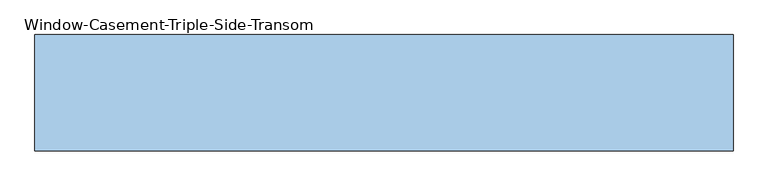
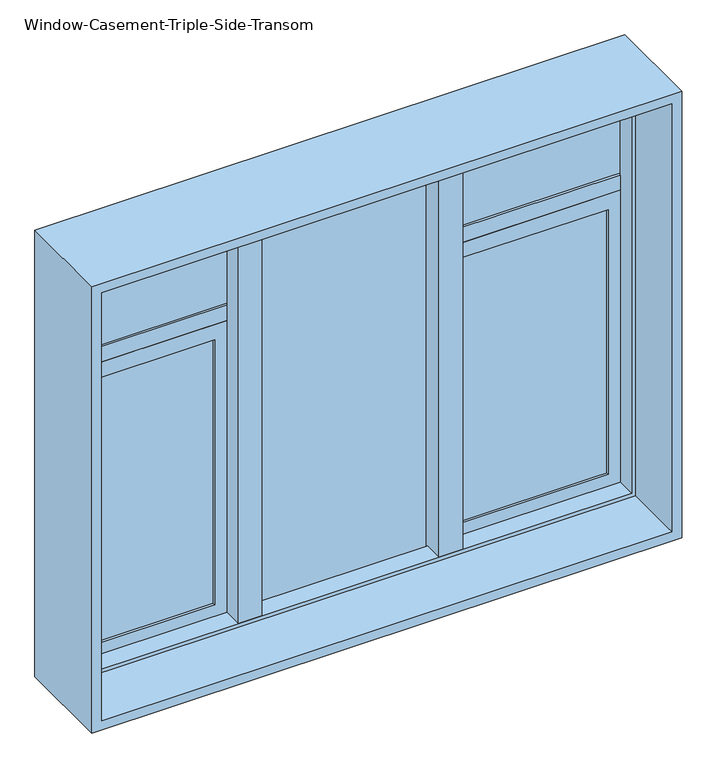
"""IFC4 building model written with IfcOpenShell, lengths in millimetres: window geometry, Window-Casement-Triple-Side-Transom : 5'*4' Window."""

import ifcopenshell
import ifcopenshell.guid

model = None  # the IFC model being written
_history = None  # IfcOwnerHistory: only IFC2X3 demands one
_inside = {}  # id of a spatial element -> (the spatial element, [elements in it])
_under = {}  # id of a project, library or spatial element -> (it, [spatial elements below it])
_declared = {}  # id of a project -> (the project, [libraries it declares])
_typed = {}  # id of a type object -> (the type object, [elements of that type])
_made_of = {}  # id of a material, layer set ... -> (it, [elements and type objects made of it])


def new_model(schema):
    """Start an empty IFC model of exactly this schema.

    Asked for "IFC4X3", IfcOpenShell would pick the latest addendum, in which some entities
    have other attributes; the version numbers below select the first issue.
    IFC2X3 requires an IfcOwnerHistory on every rooted entity: one is made here for all.
    """
    global model, _history
    if schema == "IFC4X3":
        model = ifcopenshell.file(schema_version=(4, 3, 0, 0))
    else:
        model = ifcopenshell.file(schema=schema)
    _inside.clear()
    _under.clear()
    _declared.clear()
    _typed.clear()
    _made_of.clear()
    _history = None
    if model.schema == "IFC2X3":
        org = make("IfcOrganization", Name="unknown")
        user = make(
            "IfcPersonAndOrganization",
            ThePerson=make("IfcPerson", FamilyName="unknown"),
            TheOrganization=org,
        )
        app = make(
            "IfcApplication",
            ApplicationDeveloper=org,
            Version="unknown",
            ApplicationFullName="unknown",
            ApplicationIdentifier="unknown",
        )
        _history = make(
            "IfcOwnerHistory",
            OwningUser=user,
            OwningApplication=app,
            ChangeAction="ADDED",
            CreationDate=0,
        )
    return model


def make(cls, **values):
    """One entity of the class cls with the attributes given. An attribute that is None is left unset."""
    return model.create_entity(
        cls, **{name: value for name, value in values.items() if value is not None}
    )


def rooted(cls, **values):
    """An entity with a GlobalId (a new one), such as an element, a storey or a relation."""
    return make(cls, GlobalId=ifcopenshell.guid.new(), OwnerHistory=_history, **values)


def si_unit(unit_type, name, prefix=None):
    """IfcSIUnit, for example si_unit("LENGTHUNIT", "METRE", prefix="MILLI")."""
    return make("IfcSIUnit", UnitType=unit_type, Prefix=prefix, Name=name)


def assignment(units):
    """IfcUnitAssignment: the units of a project."""
    return None if units is None else make("IfcUnitAssignment", Units=units)


def point(xyz):
    """IfcCartesianPoint."""
    return None if xyz is None else make("IfcCartesianPoint", Coordinates=xyz)


def direction(xyz):
    """IfcDirection."""
    return None if xyz is None else make("IfcDirection", DirectionRatios=xyz)


def frame(location, z_axis=None, x_axis=None):
    """IfcAxis2Placement3D, a coordinate frame: its origin and axes. An axis left out is left unset."""
    return make(
        "IfcAxis2Placement3D",
        Location=point(location),
        Axis=direction(z_axis),
        RefDirection=direction(x_axis),
    )


def origin():
    """The frame at (0, 0, 0) with its axes left unset."""
    return frame((0.0, 0.0, 0.0))


def place(relative_to, where):
    """IfcLocalPlacement: puts the frame where relative to a parent placement (None: the world)."""
    return make(
        "IfcLocalPlacement", PlacementRelTo=relative_to, RelativePlacement=where
    )


def context(
    kind, dimensions, precision=None, world=None, true_north=None, identifier=None
):
    """IfcGeometricRepresentationContext, for example the 3D "Model" context."""
    return make(
        "IfcGeometricRepresentationContext",
        ContextIdentifier=identifier,
        ContextType=kind,
        CoordinateSpaceDimension=dimensions,
        Precision=precision,
        WorldCoordinateSystem=world,
        TrueNorth=true_north,
    )


def project(units=None, contexts=None):
    """IfcProject with its units and contexts."""
    return rooted(
        "IfcProject",
        Name="project",
        RepresentationContexts=contexts,
        UnitsInContext=assignment(units),
    )


def spatial(cls, under=None, at=None, **own):
    """A site, building, storey or space (cls), placed at a placement, below another one or the project."""
    s = rooted(cls, ObjectPlacement=at, **own)
    if under is not None:
        _under.setdefault(under.id(), (under, []))[1].append(s)
    return s


def polyline(points):
    """IfcPolyline through the points."""
    return make("IfcPolyline", Points=[point(p) for p in points])


def outline(outer, holes=None, kind="AREA"):
    """IfcArbitraryClosedProfileDef: a profile drawn as a closed curve; with holes, ...WithVoids."""
    if holes is None:
        return make("IfcArbitraryClosedProfileDef", ProfileType=kind, OuterCurve=outer)
    return make(
        "IfcArbitraryProfileDefWithVoids",
        ProfileType=kind,
        OuterCurve=outer,
        InnerCurves=holes,
    )


def extrude(swept, where, along, depth):
    """IfcExtrudedAreaSolid: the profile swept, set in the frame where, extruded along a direction by depth."""
    return make(
        "IfcExtrudedAreaSolid",
        SweptArea=swept,
        Position=where,
        ExtrudedDirection=direction(along),
        Depth=depth,
    )


def faces_of(points, faces, orient=None, outer=None):
    """IfcFace entities. A face is a list of loops; a loop is a list of indices into points, from 0.

    orient and outer hold one flag for each loop. By default every Orientation is true, the
    first loop of a face is its IfcFaceOuterBound and the others are IfcFaceBound.
    """
    made = []
    for i, loops in enumerate(faces):
        bounds = []
        for j, loop in enumerate(loops):
            is_outer = j == 0 if outer is None else outer[i][j]
            bounds.append(
                make(
                    "IfcFaceOuterBound" if is_outer else "IfcFaceBound",
                    Bound=make("IfcPolyLoop", Polygon=[points[k] for k in loop]),
                    Orientation=True if orient is None else orient[i][j],
                )
            )
        made.append(make("IfcFace", Bounds=bounds))
    return made


def faceted_brep(points, faces, orient=None, outer=None, voids=None):
    """IfcFacetedBrep: a solid bounded by flat faces; with voids (closed shells), ...WithVoids."""
    shared = [point(p) for p in points]
    hull = make("IfcClosedShell", CfsFaces=faces_of(shared, faces, orient, outer))
    if voids is None:
        return make("IfcFacetedBrep", Outer=hull)
    return make(
        "IfcFacetedBrepWithVoids",
        Outer=hull,
        Voids=[
            make(cls, CfsFaces=faces_of(shared, fs, o, b)) for cls, fs, o, b in voids
        ],
    )


def shape(context_of_items, identifier, shape_type, items):
    """IfcShapeRepresentation: the items that make up one representation, for example the "Body"."""
    return make(
        "IfcShapeRepresentation",
        ContextOfItems=context_of_items,
        RepresentationIdentifier=identifier,
        RepresentationType=shape_type,
        Items=items,
    )


def source(mapping_origin, context_of_items, identifier, shape_type, items):
    """IfcRepresentationMap: a shape defined once, which mapped items show again and again."""
    return make(
        "IfcRepresentationMap",
        MappingOrigin=mapping_origin,
        MappedRepresentation=shape(context_of_items, identifier, shape_type, items),
    )


def transform(
    local_origin,
    x_axis=None,
    y_axis=None,
    z_axis=None,
    scale=None,
    scale2=None,
    scale3=None,
    uniform=True,
):
    """IfcCartesianTransformationOperator3D, or its non-uniform kind. x_axis, y_axis, z_axis: its Axis1, 2, 3."""
    if uniform:
        return make(
            "IfcCartesianTransformationOperator3D",
            Axis1=direction(x_axis),
            Axis2=direction(y_axis),
            LocalOrigin=point(local_origin),
            Scale=scale,
            Axis3=direction(z_axis),
        )
    return make(
        "IfcCartesianTransformationOperator3DnonUniform",
        Axis1=direction(x_axis),
        Axis2=direction(y_axis),
        LocalOrigin=point(local_origin),
        Scale=scale,
        Axis3=direction(z_axis),
        Scale2=scale2,
        Scale3=scale3,
    )


def mapped(mapping_source, mapping_target):
    """IfcMappedItem: shows the shape of a source again, moved by a transform."""
    return make(
        "IfcMappedItem", MappingSource=mapping_source, MappingTarget=mapping_target
    )


def made_of(thing, what):
    """Note that an element or type object is made of a material, layer set ...; save() writes the relation."""
    if what is not None:
        _made_of.setdefault(what.id(), (what, []))[1].append(thing)
    return thing


def element(
    cls,
    number,
    at=None,
    inside=None,
    cuts=None,
    type_object=None,
    material=None,
    context=None,
    identifier="Body",
    shape_type=None,
    held_by="IfcProductDefinitionShape",
    body=None,
    shapes=None,
    **own,
):
    """One element of the class cls, such as IfcWall. Its Tag is "e" and its number.

    at: its placement. inside: the storey or other place that contains it. cuts: it is an
    opening in that element (IfcRelVoidsElement). A single representation is given by context,
    identifier, shape_type and body (its items); several are given by shapes. held_by: the class
    of the entity that holds the representations. save() writes the other relations.
    """
    e = rooted(cls, Tag="e%d" % number, ObjectPlacement=at, **own)
    if body is not None:
        shapes = [shape(context, identifier, shape_type, body)]
    if shapes is not None:
        e.Representation = make(held_by, Representations=shapes)
    if inside is not None:
        _inside.setdefault(inside.id(), (inside, []))[1].append(e)
    if cuts is not None:
        rooted(
            "IfcRelVoidsElement", RelatingBuildingElement=cuts, RelatedOpeningElement=e
        )
    if type_object is not None:
        _typed.setdefault(type_object.id(), (type_object, []))[1].append(e)
    return made_of(e, material)


def aggregate(whole, parts):
    """IfcRelAggregates: a whole, such as a stair, and the parts it consists of."""
    return rooted("IfcRelAggregates", RelatingObject=whole, RelatedObjects=parts)


def save(model, path):
    """Write the relations noted so far, then the file.

    IfcRelAggregates (storeys below a building ...), IfcRelContainedInSpatialStructure (elements
    in a storey), IfcRelDefinesByType, IfcRelAssociatesMaterial and IfcRelDeclares: one each for
    every whole, place, type object, material and project.
    """
    for whole, parts in _under.values():
        aggregate(whole, parts)
    for where, things in _inside.values():
        rooted(
            "IfcRelContainedInSpatialStructure",
            RelatedElements=things,
            RelatingStructure=where,
        )
    for kind, things in _typed.values():
        rooted("IfcRelDefinesByType", RelatedObjects=things, RelatingType=kind)
    for what, things in _made_of.values():
        rooted("IfcRelAssociatesMaterial", RelatedObjects=things, RelatingMaterial=what)
    for by, libraries in _declared.values():
        rooted("IfcRelDeclares", RelatingContext=by, RelatedDefinitions=libraries)
    model.write(path)


def window_casement_triple_side_transom_94e0c3a0(model_context):
    return source(origin(), model_context, "Body", "SolidModel", [
        faceted_brep([(-736.6, 85.725, 1955.8), (-736.6, 127.0, 1955.8), (736.6, 127.0, 1955.8), (736.6, 85.725, 1955.8), (-726.4796875, 34.925, 1945.6796875), (-726.4796875, 85.725, 1945.6796875), (726.4796875, 85.725, 1945.6796875), (726.4796875, 34.925, 1945.6796875), (-736.6, -127.0, 1955.8), (-736.6, 34.925, 1955.8), (736.6, 34.925, 1955.8), (736.6, -127.0, 1955.8), (-762.0, 127.0, 1981.2), (-762.0, -127.0, 1981.2), (762.0, -127.0, 1981.2), (762.0, 127.0, 1981.2), (736.6, 127.0, 787.4), (736.6, 85.725, 787.4), (726.4796875, 85.725, 797.5203125), (726.4796875, 34.925, 797.5203125), (736.6, 34.925, 787.4), (736.6, -127.0, 787.4), (762.0, -127.0, 762.0), (762.0, 127.0, 762.0), (-736.6, 127.0, 787.4), (-736.6, 85.725, 787.4), (-726.4796875, 85.725, 797.5203125), (-726.4796875, 34.925, 797.5203125), (-736.6, 34.925, 787.4), (-736.6, -127.0, 787.4), (-762.0, -127.0, 762.0), (-762.0, 127.0, 762.0)], [[[0, 1, 2, 3]], [[4, 5, 6, 7]], [[8, 9, 10, 11]], [[12, 13, 14, 15]], [[3, 2, 16, 17]], [[7, 6, 18, 19]], [[11, 10, 20, 21]], [[15, 14, 22, 23]], [[17, 16, 24, 25]], [[19, 18, 26, 27]], [[21, 20, 28, 29]], [[23, 22, 30, 31]], [[25, 24, 1, 0]], [[3, 17, 25, 0], [5, 26, 18, 6]], [[27, 26, 5, 4]], [[9, 28, 20, 10], [7, 19, 27, 4]], [[29, 28, 9, 8]], [[13, 30, 22, 14], [11, 21, 29, 8]], [[31, 30, 13, 12]], [[15, 23, 31, 12], [1, 24, 16, 2]]]),
        extrude(outline(polyline([(-228.6, 123.825), (-228.6, 34.925), (-289.5203125, 34.925), (-289.5203125, 85.725), (-279.4, 85.725), (-279.4, 123.825), (-228.6, 123.825)])), frame((0.0, 0.0, 787.4), z_axis=(0.0, 0.0, 1.0), x_axis=(1.0, 0.0, 0.0)), (0.0, 0.0, 1.0), 1168.4),
        extrude(outline(polyline([(279.4, 123.825), (279.4, 85.725), (289.5203125, 85.725), (289.5203125, 34.925), (228.6, 34.925), (228.6, 123.825), (279.4, 123.825)])), frame((0.0, 0.0, 787.4), z_axis=(0.0, 0.0, 1.0), x_axis=(1.0, 0.0, 0.0)), (0.0, 0.0, 1.0), 1168.4),
        extrude(outline(polyline([(1594.5048438, 279.4), (787.4, 279.4), (787.4, 736.6), (1594.5048438, 736.6), (1594.5048438, 279.4)]), holes=[polyline([(1552.6345313, 694.7296875), (829.2703125, 694.7296875), (829.2703125, 321.2703125), (1552.6345313, 321.2703125), (1552.6345313, 694.7296875)])]), frame((0.0, 85.725, 0.0), z_axis=(0.0, 1.0, 0.0), x_axis=(0.0, 0.0, 1.0)), (0.0, 0.0, 1.0), 31.75),
        extrude(outline(polyline([(1594.5048438, -736.6), (787.4, -736.6), (787.4, -279.4), (1594.5048438, -279.4), (1594.5048438, -736.6)]), holes=[polyline([(1552.6345313, -321.2703125), (829.2703125, -321.2703125), (829.2703125, -694.7296875), (1552.6345313, -694.7296875), (1552.6345313, -321.2703125)])]), frame((0.0, 85.725, 0.0), z_axis=(0.0, 1.0, 0.0), x_axis=(0.0, 0.0, 1.0)), (0.0, 0.0, 1.0), 31.75),
        extrude(outline(polyline([(-321.2703125, 111.125), (-321.2703125, 104.775), (-694.7296875, 104.775), (-694.7296875, 111.125), (-321.2703125, 111.125)])), frame((0.0, 0.0, 829.2703125), z_axis=(0.0, 0.0, 1.0), x_axis=(1.0, 0.0, 0.0)), (0.0, 0.0, 1.0), 723.3642188),
        extrude(outline(polyline([(-321.2703125, 98.425), (-321.2703125, 92.075), (-694.7296875, 92.075), (-694.7296875, 98.425), (-321.2703125, 98.425)])), frame((0.0, 0.0, 829.2703125), z_axis=(0.0, 0.0, 1.0), x_axis=(1.0, 0.0, 0.0)), (0.0, 0.0, 1.0), 723.3642188),
        extrude(outline(polyline([(694.7296875, 111.125), (694.7296875, 104.775), (321.2703125, 104.775), (321.2703125, 111.125), (694.7296875, 111.125)])), frame((0.0, 0.0, 829.2703125), z_axis=(0.0, 0.0, 1.0), x_axis=(1.0, 0.0, 0.0)), (0.0, 0.0, 1.0), 723.3642188),
        extrude(outline(polyline([(694.7296875, 98.425), (694.7296875, 92.075), (321.2703125, 92.075), (321.2703125, 98.425), (694.7296875, 98.425)])), frame((0.0, 0.0, 829.2703125), z_axis=(0.0, 0.0, 1.0), x_axis=(1.0, 0.0, 0.0)), (0.0, 0.0, 1.0), 723.3642188),
        extrude(outline(polyline([(736.6, 117.475), (736.6, 85.725), (279.4, 85.725), (279.4, 117.475), (736.6, 117.475)])), frame((0.0, 0.0, 1594.5048438), z_axis=(0.0, 0.0, 1.0), x_axis=(1.0, 0.0, 0.0)), (0.0, 0.0, 1.0), 41.8703125),
        extrude(outline(polyline([(228.6, 111.125), (228.6, 104.775), (-228.6, 104.775), (-228.6, 111.125), (228.6, 111.125)])), frame((0.0, 0.0, 787.4), z_axis=(0.0, 0.0, 1.0), x_axis=(1.0, 0.0, 0.0)), (0.0, 0.0, 1.0), 1168.4),
        extrude(outline(polyline([(228.6, 98.425), (228.6, 92.075), (-228.6, 92.075), (-228.6, 98.425), (228.6, 98.425)])), frame((0.0, 0.0, 787.4), z_axis=(0.0, 0.0, 1.0), x_axis=(1.0, 0.0, 0.0)), (0.0, 0.0, 1.0), 1168.4),
        extrude(outline(polyline([(-279.4, 117.475), (-279.4, 85.725), (-736.6, 85.725), (-736.6, 117.475), (-279.4, 117.475)])), frame((0.0, 0.0, 1594.5048438), z_axis=(0.0, 0.0, 1.0), x_axis=(1.0, 0.0, 0.0)), (0.0, 0.0, 1.0), 41.8703125),
        extrude(outline(polyline([(-279.4, 111.125), (-279.4, 104.775), (-736.6, 104.775), (-736.6, 111.125), (-279.4, 111.125)])), frame((0.0, 0.0, 1636.3751563), z_axis=(0.0, 0.0, 1.0), x_axis=(1.0, 0.0, 0.0)), (0.0, 0.0, 1.0), 319.4248438),
        extrude(outline(polyline([(-279.4, 98.425), (-279.4, 92.075), (-736.6, 92.075), (-736.6, 98.425), (-279.4, 98.425)])), frame((0.0, 0.0, 1636.3751563), z_axis=(0.0, 0.0, 1.0), x_axis=(1.0, 0.0, 0.0)), (0.0, 0.0, 1.0), 319.4248438),
        extrude(outline(polyline([(736.6, 111.125), (736.6, 104.775), (279.4, 104.775), (279.4, 111.125), (736.6, 111.125)])), frame((0.0, 0.0, 1636.3751563), z_axis=(0.0, 0.0, 1.0), x_axis=(1.0, 0.0, 0.0)), (0.0, 0.0, 1.0), 319.4248438),
        extrude(outline(polyline([(736.6, 98.425), (736.6, 92.075), (279.4, 92.075), (279.4, 98.425), (736.6, 98.425)])), frame((0.0, 0.0, 1636.3751563), z_axis=(0.0, 0.0, 1.0), x_axis=(1.0, 0.0, 0.0)), (0.0, 0.0, 1.0), 319.4248438),
    ])


if __name__ == "__main__":
    model = new_model("IFC4")
    model_context = context("Model", 3, world=origin())
    ifc_project = project(units=[si_unit("LENGTHUNIT", "METRE", prefix="MILLI")], contexts=[model_context])
    site = spatial("IfcSite", under=ifc_project)
    building = spatial("IfcBuilding", under=site)
    placement = place(None, origin())
    window_casement_triple_side_transom_shape = window_casement_triple_side_transom_94e0c3a0(model_context)
    element("IfcWindow", 1, ObjectType="Window-Casement-Triple-Side-Transom : 5'*4' Window", at=placement, inside=building, context=model_context, shape_type="MappedRepresentation", body=[
        mapped(window_casement_triple_side_transom_shape, transform((0.0, 0.0, 0.0), x_axis=(1.0, 0.0, 0.0), y_axis=(0.0, 1.0, 0.0), z_axis=(0.0, 0.0, 1.0))),
    ])
    save(model, "model.ifc")

# Revit data of these elements
# Type "Window-Casement-Triple-Side-Transom : 5'*4' Window"
#   Type Mark = "21"
#   Fire Rating = "0.5h"
#   Assembly Code = "B2020100"
#   Analytic Construction = "Double glazing - domestic"
#   Window Width = 1' - 8"
#   Window Inset [instance default] = 0' - 0 5/8"
#   Wall Thickness [instance default] = 0' - 6"
#   Visual Light Transmittance = 0.81
#   Transom Height Ratio = 0.3
#   Thermal Resistance (R) = 1.8146 (h·ft²·°F)/BTU
#   Solar Heat Gain Coefficient = 0.76
#   Rough Width = 5' - 0 1/2"
#   Rough Height = 4' - 0 1/2"
#   Open Window Height = 2' - 9.6"
#   Heat Transfer Coefficient (U) = 0.5511 BTU/(h·ft²·°F)
#   Height = 4' - 0"
#   Transom Height = 1' - 2.4"
#   Frame Gap 3 [instance default] = 0' - 1 83/128"
#   Frame Gap 2 [instance default] = 0' - 0 5/8"
#   Frame Gap 1 = 0' - 1 51/128"
#   Default Sill Height = 2' - 6"
#   Width = 5' - 0"
#   Frame Material = Metal - Aluminum
#   Glass Panel Material = Glass
#   Wall Closure = (empty or 0)
# Element 1 (IfcWindow, "Window-Casement-Triple-Side-Transom : 5'*4' Window")
#   Wall Thickness = 0' - 10"
#   Materials on its faces: "Metal - Aluminum", "Glass"
# Materials
#   "Metal - Aluminum": class "Metal", colour RGB 244 244 244, transparency 0, Cost = 0
#   "Glass": class "Glass", colour RGB 0 128 192, transparency 0.75, Description = "Soda Lime Glass", Cost = 0
